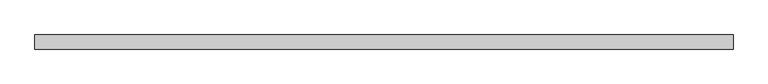
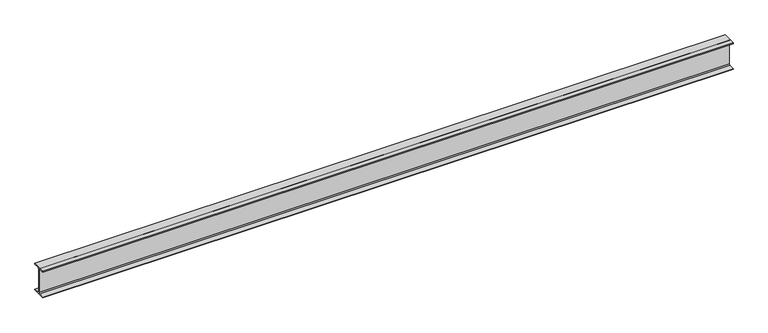
"""IFC4 building model written with IfcOpenShell, lengths in millimetres: beam geometry, 0912_Steel Framing_H-KSD3502 : H_SB_ASB_H-350x175x7x11."""

from ifc_helpers import new_model, si_unit, point, frame, frame_2d, origin, place, context, project, spatial, polyline, circle_curve, trimmed, segment, composite_curve, outline, extrude, source, transform, mapped, element, save


def beam_7a475a0c(model_context):
    return source(origin(), model_context, "Body", "SweptSolid", [
        extrude(outline(composite_curve([segment(polyline([(87.5, -164.0), (87.5, -175.0), (-87.5, -175.0), (-87.5, -164.0), (-17.5, -164.0)]), True, "CONTINUOUS"), segment(trimmed(circle_curve(frame_2d((-17.5, -150.0)), 14.0), [point((-17.5, -164.0))], [point((-3.5, -150.0))], True, "CARTESIAN"), True, "CONTINUOUS"), segment(polyline([(-3.5, -150.0), (-3.5, 150.0)]), True, "CONTINUOUS"), segment(trimmed(circle_curve(frame_2d((-17.5, 150.0)), 14.0), [point((-3.5, 150.0))], [point((-17.5, 164.0))], True, "CARTESIAN"), True, "CONTINUOUS"), segment(polyline([(-17.5, 164.0), (-87.5, 164.0), (-87.5, 175.0), (87.5, 175.0), (87.5, 164.0), (17.5, 164.0)]), True, "CONTINUOUS"), segment(trimmed(circle_curve(frame_2d((17.5, 150.0)), 14.0), [point((17.5, 164.0))], [point((3.5, 150.0))], True, "CARTESIAN"), True, "CONTINUOUS"), segment(polyline([(3.5, 150.0), (3.5, -150.0)]), True, "CONTINUOUS"), segment(trimmed(circle_curve(frame_2d((17.5, -150.0)), 14.0), [point((3.5, -150.0))], [point((17.5, -164.0))], True, "CARTESIAN"), True, "CONTINUOUS"), segment(polyline([(17.5, -164.0), (87.5, -164.0)]), True, "CONTINUOUS")], self_intersect=False)), frame((-4298.8712061, 0.0, 0.0), z_axis=(1.0, 0.0, 0.0), x_axis=(0.0, 1.0, 0.0)), (0.0, 0.0, 1.0), 8634.4837274),
    ])


if __name__ == "__main__":
    model = new_model("IFC4")
    model_context = context("Model", 3, world=origin())
    ifc_project = project(units=[si_unit("LENGTHUNIT", "METRE", prefix="MILLI")], contexts=[model_context])
    site = spatial("IfcSite", under=ifc_project)
    building = spatial("IfcBuilding", under=site)
    placement = place(None, origin())
    beam_shape = beam_7a475a0c(model_context)
    element("IfcBeam", 1, ObjectType="0912_Steel Framing_H-KSD3502 : H_SB_ASB_H-350x175x7x11", at=placement, inside=building, context=model_context, shape_type="MappedRepresentation", body=[
        mapped(beam_shape, transform((0.0, 0.0, 0.0), x_axis=(1.0, 0.0, 0.0), y_axis=(0.0, 1.0, 0.0), z_axis=(0.0, 0.0, 1.0))),
    ])
    save(model, "model.ifc")

# Revit data of these elements
# Type "0912_Steel Framing_H-KSD3502 : H_SB_ASB_H-350x175x7x11"
#   H_WM Code_1 = "S01AA002-00001 | Main Steel Structure Fabrication Work | Shelter/Building | Medium Steel - Standard (90KG/M>Weight≥30KG/M) | Material: (   )"
#   H_WM Code_2 = "S03AA028-00001 | Main Steel Structure Erection Work | Shelter/Building | Medium Steel (90KG/M>Weight≥30KG/M) | Material: (   )"
#   H_WM Code_3 = "S01AA010-00001 | Main Steel Structure Fabrication Work | Shelter/Building | Steel Painting/Coating | for Non-Fireproofed Steel Surface, Surface Preparation, Primer, Second & Final Coat | Material: (   )"
#   H_Q'ty Cal Type Tag = "SB-Q2"
#   Width = 17.5 cm
#   Web Thickness = 0.7 cm
#   Web Fillet = 1.4 cm
#   Warping Constant = 282000.0 cm⁶
#   W = 0
#   Torsional Moment of Inertia = 19.4042 cm⁴
#   Section Area = 63.14 cm²
#   Plastic Modulus weak axis = 174.0 cm³
#   Plastic Modulus strong axis = 868.0 cm³
#   Perimeter = 1.36 m²/m
#   Nominal Weight = 49.60 kgf/m
#   Moment of Inertia weak axis = 984.00 cm⁴
#   Moment of Inertia strong axis = 13600.00 cm⁴
#   Height = 35.0 cm
#   Flange Thickness = 1.1 cm
#   Elastic Modulus weak axis = 112.0 cm³
#   Elastic Modulus strong axis = 775.0 cm³
#   Centroid Vertical = 17.5 cm
#   Centroid Horizontal = 8.75 cm
#   Ix = 136000000
#   Length [instance default] = 1.5240 m
#   Zx = 868000
#   b = 0.1750 m
#   h = 0.3500 m
#   r = 0.0140 m
#   s = 0.0070 m
#   t = 0.0110 m
#   A = 0.006314 m²
#   Structural Material [instance default] = Steel, 45-345
#   Assembly Code = ""
# Element 1 (IfcBeam, "0912_Steel Framing_H-KSD3502 : H_SB_ASB_H-350x175x7x11")
#   Structural Material = none
# Materials
#   "Steel, 45-345": class "Metal", colour RGB 189 187 185, transparency 0, Description = "Steel 345 MPa", Cost = 0
